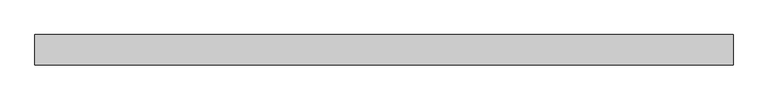
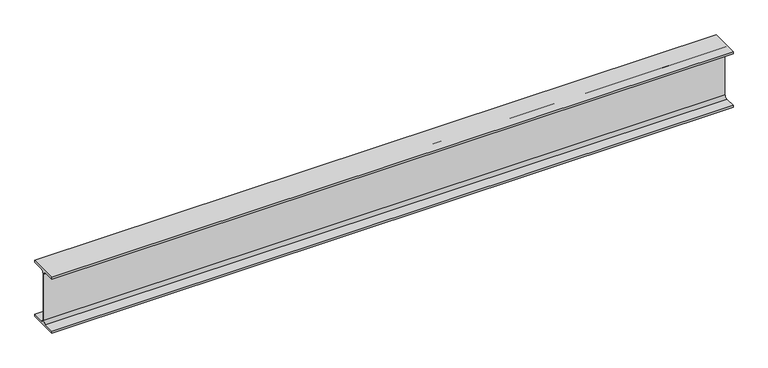
"""IFC4 building model written with IfcOpenShell, lengths in millimetres: beam geometry, 0912_Steel Framing_H-KSD3502 : H_SB_ASB_H-250x125x6x9."""

from ifc_helpers import new_model, si_unit, point, frame, frame_2d, origin, place, context, project, spatial, polyline, circle_curve, trimmed, segment, composite_curve, outline, extrude, source, transform, mapped, element, save


def beam_3295fd40(model_context):
    return source(origin(), model_context, "Body", "SweptSolid", [
        extrude(outline(composite_curve([segment(polyline([(62.5, -116.0), (62.5, -125.0), (-62.5, -125.0), (-62.5, -116.0), (-15.0, -116.0)]), True, "CONTINUOUS"), segment(trimmed(circle_curve(frame_2d((-15.0, -104.0)), 12.0), [point((-15.0, -116.0))], [point((-3.0, -104.0))], True, "CARTESIAN"), True, "CONTINUOUS"), segment(polyline([(-3.0, -104.0), (-3.0, 104.0)]), True, "CONTINUOUS"), segment(trimmed(circle_curve(frame_2d((-15.0, 104.0)), 12.0), [point((-3.0, 104.0))], [point((-15.0, 116.0))], True, "CARTESIAN"), True, "CONTINUOUS"), segment(polyline([(-15.0, 116.0), (-62.5, 116.0), (-62.5, 125.0), (62.5, 125.0), (62.5, 116.0), (15.0, 116.0)]), True, "CONTINUOUS"), segment(trimmed(circle_curve(frame_2d((15.0, 104.0)), 12.0), [point((15.0, 116.0))], [point((3.0, 104.0))], True, "CARTESIAN"), True, "CONTINUOUS"), segment(polyline([(3.0, 104.0), (3.0, -104.0)]), True, "CONTINUOUS"), segment(trimmed(circle_curve(frame_2d((15.0, -104.0)), 12.0), [point((3.0, -104.0))], [point((15.0, -116.0))], True, "CARTESIAN"), True, "CONTINUOUS"), segment(polyline([(15.0, -116.0), (62.5, -116.0)]), True, "CONTINUOUS")], self_intersect=False)), frame((-1487.2999994, 0.0, 0.0), z_axis=(1.0, 0.0, 0.0), x_axis=(0.0, 1.0, 0.0)), (0.0, 0.0, 1.0), 2892.0999994),
    ])


if __name__ == "__main__":
    model = new_model("IFC4")
    model_context = context("Model", 3, world=origin())
    ifc_project = project(units=[si_unit("LENGTHUNIT", "METRE", prefix="MILLI")], contexts=[model_context])
    site = spatial("IfcSite", under=ifc_project)
    building = spatial("IfcBuilding", under=site)
    placement = place(None, origin())
    beam_shape = beam_3295fd40(model_context)
    element("IfcBeam", 1, ObjectType="0912_Steel Framing_H-KSD3502 : H_SB_ASB_H-250x125x6x9", at=placement, inside=building, context=model_context, shape_type="MappedRepresentation", body=[
        mapped(beam_shape, transform((0.0, 0.0, 0.0), x_axis=(1.0, 0.0, 0.0), y_axis=(0.0, 1.0, 0.0), z_axis=(0.0, 0.0, 1.0))),
    ])
    save(model, "model.ifc")

# Revit data of these elements
# Type "0912_Steel Framing_H-KSD3502 : H_SB_ASB_H-250x125x6x9"
#   H_WM Code_1 = "S01AA003-00001 | Main Steel Structure Fabrication Work | Shelter/Building | Light Steel - Standard (30KG/M>Weight) | Material: (   )"
#   H_WM Code_2 = "S03AA029-00001 | Main Steel Structure Erection Work | Shelter/Building | Light Steel (30KG/M>Weight) | Material: (   )"
#   H_WM Code_3 = "S01AA010-00001 | Main Steel Structure Fabrication Work | Shelter/Building | Steel Painting/Coating | for Non-Fireproofed Steel Surface, Surface Preparation, Primer, Second & Final Coat | Material: (   )"
#   H_Q'ty Cal Type Tag = "SB-Q2"
#   Width = 12.5 cm
#   Web Thickness = 0.6 cm
#   Web Fillet = 1.2 cm
#   Warping Constant = 42539.8 cm⁶
#   W = 0
#   Torsional Moment of Inertia = 7.8102 cm⁴
#   Section Area = 37.66 cm²
#   Plastic Modulus weak axis = 73.1 cm³
#   Plastic Modulus strong axis = 366.0 cm³
#   Perimeter = 0.97 m²/m
#   Nominal Weight = 29.60 kgf/m
#   Moment of Inertia weak axis = 294.00 cm⁴
#   Moment of Inertia strong axis = 4050.00 cm⁴
#   Height = 25.0 cm
#   Flange Thickness = 0.9 cm
#   Elastic Modulus weak axis = 47.0 cm³
#   Elastic Modulus strong axis = 324.0 cm³
#   Centroid Vertical = 12.5 cm
#   Centroid Horizontal = 6.25 cm
#   Ix = 40500000
#   Length [instance default] = 1.5240 m
#   Zx = 366000
#   b = 0.1250 m
#   h = 0.2500 m
#   r = 0.0120 m
#   s = 0.0060 m
#   t = 0.0090 m
#   A = 0.003766 m²
#   Structural Material [instance default] = Steel, 45-345
#   Assembly Code = ""
# Element 1 (IfcBeam, "0912_Steel Framing_H-KSD3502 : H_SB_ASB_H-250x125x6x9")
#   Structural Material = none
# Materials
#   "Steel, 45-345": class "Metal", colour RGB 189 187 185, transparency 0, Description = "Steel 345 MPa", Cost = 0
